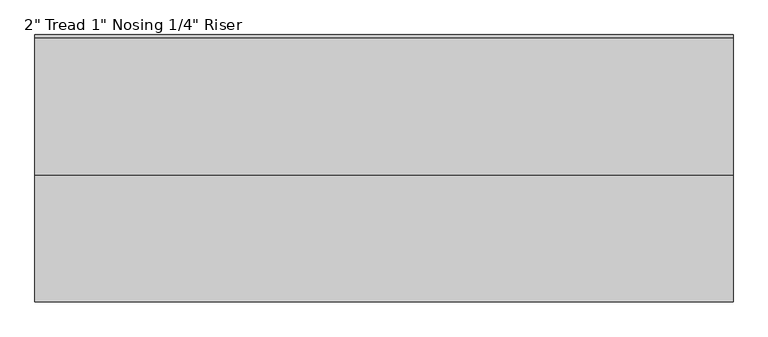
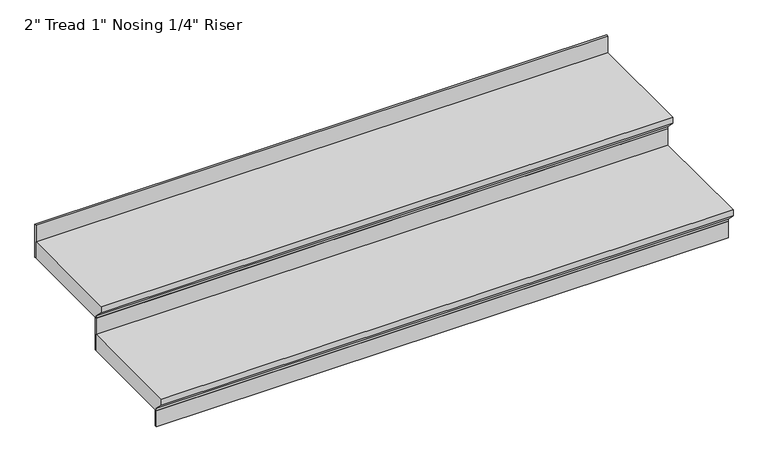
"""IFC4 building model written with IfcOpenShell, lengths in millimetres: stair flight geometry."""

from ifc_helpers import new_model, si_unit, frame, origin, place, context, project, spatial, polyline, outline, extrude, source, transform, mapped, element, save


def stair_flight_98d98def(model_context):
    return source(origin(), model_context, "Body", "SweptSolid", [
        extrude(outline(polyline([(12936.5159596, -381.0), (13266.7159596, -381.0), (13266.7159596, -431.8), (12961.9159596, -431.8), (12961.9159596, -425.45), (12936.5159596, -400.05), (12936.5159596, -381.0)])), frame((15562.1846541, 0.0, 0.0), z_axis=(1.0, 0.0, 0.0), x_axis=(0.0, 1.0, 0.0)), (0.0, 0.0, 1.0), 1674.0660814),
        extrude(outline(polyline([(17236.2507355, 12968.2659596), (17236.2507355, 12961.9159596), (15562.1846541, 12961.9159596), (15562.1846541, 12968.2659596), (17236.2507355, 12968.2659596)])), frame((0.0, 0.0, -482.6), z_axis=(0.0, 0.0, 1.0), x_axis=(1.0, 0.0, 0.0)), (0.0, 0.0, 1.0), 50.8),
        extrude(outline(polyline([(17236.2507355, 13273.0659596), (17236.2507355, 13266.7159596), (15562.1846541, 13266.7159596), (15562.1846541, 13273.0659596), (17236.2507355, 13273.0659596)])), frame((0.0, 0.0, -431.8), z_axis=(0.0, 0.0, 1.0), x_axis=(1.0, 0.0, 0.0)), (0.0, 0.0, 1.0), 101.6),
        extrude(outline(polyline([(13241.3159596, -279.4), (13571.5159596, -279.4), (13571.5159596, -330.2), (13266.7159596, -330.2), (13266.7159596, -323.85), (13241.3159596, -298.45), (13241.3159596, -279.4)])), frame((15562.1846541, 0.0, 0.0), z_axis=(1.0, 0.0, 0.0), x_axis=(0.0, 1.0, 0.0)), (0.0, 0.0, 1.0), 1674.0660814),
        extrude(outline(polyline([(17236.2507355, 13577.8659596), (17236.2507355, 13571.5159596), (15562.1846541, 13571.5159596), (15562.1846541, 13577.8659596), (17236.2507355, 13577.8659596)])), frame((0.0, 0.0, -330.2), z_axis=(0.0, 0.0, 1.0), x_axis=(1.0, 0.0, 0.0)), (0.0, 0.0, 1.0), 101.6),
    ])


if __name__ == "__main__":
    model = new_model("IFC4")
    model_context = context("Model", 3, world=origin())
    ifc_project = project(units=[si_unit("LENGTHUNIT", "METRE", prefix="MILLI")], contexts=[model_context])
    site = spatial("IfcSite", under=ifc_project)
    building = spatial("IfcBuilding", under=site)
    placement = place(None, origin())
    stair_flight_shape = stair_flight_98d98def(model_context)
    element("IfcStairFlight", 1, ObjectType="2\" Tread 1\" Nosing 1/4\" Riser", at=placement, inside=building, context=model_context, shape_type="MappedRepresentation", body=[
        mapped(stair_flight_shape, transform((0.0, 0.0, 0.0), x_axis=(1.0, 0.0, 0.0), y_axis=(0.0, 1.0, 0.0), z_axis=(0.0, 0.0, 1.0))),
    ])
    save(model, "model.ifc")
